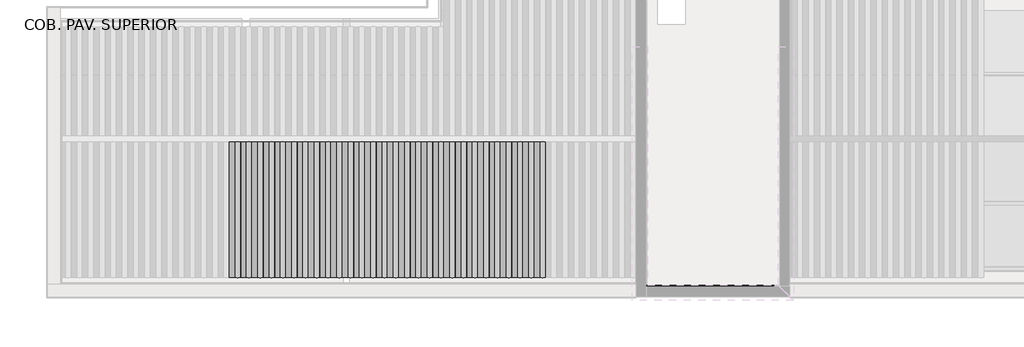
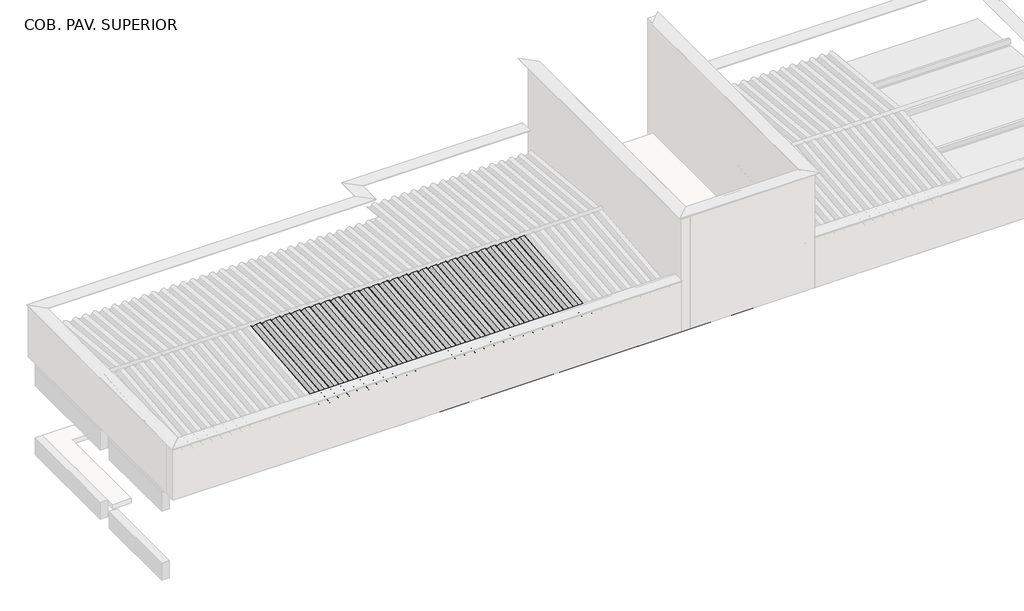
# One storey, part 2 of 7: 38 beams, 9 columns.
"""IFC4 building model written with IfcOpenShell, lengths in millimetres."""

import ifcopenshell
import ifcopenshell.guid

model = None  # the IFC model being written
_history = None  # IfcOwnerHistory: only IFC2X3 demands one
_inside = {}  # id of a spatial element -> (the spatial element, [elements in it])
_under = {}  # id of a project, library or spatial element -> (it, [spatial elements below it])
_declared = {}  # id of a project -> (the project, [libraries it declares])
_typed = {}  # id of a type object -> (the type object, [elements of that type])
_made_of = {}  # id of a material, layer set ... -> (it, [elements and type objects made of it])


def new_model(schema):
    """Start an empty IFC model of exactly this schema.

    Asked for "IFC4X3", IfcOpenShell would pick the latest addendum, in which some entities
    have other attributes; the version numbers below select the first issue.
    IFC2X3 requires an IfcOwnerHistory on every rooted entity: one is made here for all.
    """
    global model, _history
    if schema == "IFC4X3":
        model = ifcopenshell.file(schema_version=(4, 3, 0, 0))
    else:
        model = ifcopenshell.file(schema=schema)
    _inside.clear()
    _under.clear()
    _declared.clear()
    _typed.clear()
    _made_of.clear()
    _history = None
    if model.schema == "IFC2X3":
        org = make("IfcOrganization", Name="unknown")
        user = make(
            "IfcPersonAndOrganization",
            ThePerson=make("IfcPerson", FamilyName="unknown"),
            TheOrganization=org,
        )
        app = make(
            "IfcApplication",
            ApplicationDeveloper=org,
            Version="unknown",
            ApplicationFullName="unknown",
            ApplicationIdentifier="unknown",
        )
        _history = make(
            "IfcOwnerHistory",
            OwningUser=user,
            OwningApplication=app,
            ChangeAction="ADDED",
            CreationDate=0,
        )
    return model


def make(cls, **values):
    """One entity of the class cls with the attributes given. An attribute that is None is left unset."""
    return model.create_entity(
        cls, **{name: value for name, value in values.items() if value is not None}
    )


def rooted(cls, **values):
    """An entity with a GlobalId (a new one), such as an element, a storey or a relation."""
    return make(cls, GlobalId=ifcopenshell.guid.new(), OwnerHistory=_history, **values)


def si_unit(unit_type, name, prefix=None):
    """IfcSIUnit, for example si_unit("LENGTHUNIT", "METRE", prefix="MILLI")."""
    return make("IfcSIUnit", UnitType=unit_type, Prefix=prefix, Name=name)


def assignment(units):
    """IfcUnitAssignment: the units of a project."""
    return None if units is None else make("IfcUnitAssignment", Units=units)


def point(xyz):
    """IfcCartesianPoint."""
    return None if xyz is None else make("IfcCartesianPoint", Coordinates=xyz)


def direction(xyz):
    """IfcDirection."""
    return None if xyz is None else make("IfcDirection", DirectionRatios=xyz)


def frame(location, z_axis=None, x_axis=None):
    """IfcAxis2Placement3D, a coordinate frame: its origin and axes. An axis left out is left unset."""
    return make(
        "IfcAxis2Placement3D",
        Location=point(location),
        Axis=direction(z_axis),
        RefDirection=direction(x_axis),
    )


def frame_2d(location, x_axis=None):
    """IfcAxis2Placement2D, a coordinate frame in the plane: its origin and x axis."""
    return make(
        "IfcAxis2Placement2D", Location=point(location), RefDirection=direction(x_axis)
    )


def origin():
    """The frame at (0, 0, 0) with its axes left unset."""
    return frame((0.0, 0.0, 0.0))


def place(relative_to, where):
    """IfcLocalPlacement: puts the frame where relative to a parent placement (None: the world)."""
    return make(
        "IfcLocalPlacement", PlacementRelTo=relative_to, RelativePlacement=where
    )


def context(
    kind, dimensions, precision=None, world=None, true_north=None, identifier=None
):
    """IfcGeometricRepresentationContext, for example the 3D "Model" context."""
    return make(
        "IfcGeometricRepresentationContext",
        ContextIdentifier=identifier,
        ContextType=kind,
        CoordinateSpaceDimension=dimensions,
        Precision=precision,
        WorldCoordinateSystem=world,
        TrueNorth=true_north,
    )


def project(units=None, contexts=None):
    """IfcProject with its units and contexts."""
    return rooted(
        "IfcProject",
        Name="project",
        RepresentationContexts=contexts,
        UnitsInContext=assignment(units),
    )


def spatial(cls, under=None, at=None, **own):
    """A site, building, storey or space (cls), placed at a placement, below another one or the project."""
    s = rooted(cls, ObjectPlacement=at, **own)
    if under is not None:
        _under.setdefault(under.id(), (under, []))[1].append(s)
    return s


def polyline(points):
    """IfcPolyline through the points."""
    return make("IfcPolyline", Points=[point(p) for p in points])


def circle_curve(where, radius):
    """IfcCircle in the frame where."""
    return make("IfcCircle", Position=where, Radius=radius)


def trimmed(basis, trim1, trim2, sense, master):
    """IfcTrimmedCurve: the piece of a basis curve between two trims."""
    return make(
        "IfcTrimmedCurve",
        BasisCurve=basis,
        Trim1=trim1,
        Trim2=trim2,
        SenseAgreement=sense,
        MasterRepresentation=master,
    )


def segment(curve, same_sense, transition):
    """IfcCompositeCurveSegment."""
    return make(
        "IfcCompositeCurveSegment",
        Transition=transition,
        SameSense=same_sense,
        ParentCurve=curve,
    )


def composite_curve(segments, self_intersect=None):
    """IfcCompositeCurve: segments joined end to end."""
    return make("IfcCompositeCurve", Segments=segments, SelfIntersect=self_intersect)


def outline(outer, holes=None, kind="AREA"):
    """IfcArbitraryClosedProfileDef: a profile drawn as a closed curve; with holes, ...WithVoids."""
    if holes is None:
        return make("IfcArbitraryClosedProfileDef", ProfileType=kind, OuterCurve=outer)
    return make(
        "IfcArbitraryProfileDefWithVoids",
        ProfileType=kind,
        OuterCurve=outer,
        InnerCurves=holes,
    )


def extrude(swept, where, along, depth):
    """IfcExtrudedAreaSolid: the profile swept, set in the frame where, extruded along a direction by depth."""
    return make(
        "IfcExtrudedAreaSolid",
        SweptArea=swept,
        Position=where,
        ExtrudedDirection=direction(along),
        Depth=depth,
    )


def faces_of(points, faces, orient=None, outer=None):
    """IfcFace entities. A face is a list of loops; a loop is a list of indices into points, from 0.

    orient and outer hold one flag for each loop. By default every Orientation is true, the
    first loop of a face is its IfcFaceOuterBound and the others are IfcFaceBound.
    """
    made = []
    for i, loops in enumerate(faces):
        bounds = []
        for j, loop in enumerate(loops):
            is_outer = j == 0 if outer is None else outer[i][j]
            bounds.append(
                make(
                    "IfcFaceOuterBound" if is_outer else "IfcFaceBound",
                    Bound=make("IfcPolyLoop", Polygon=[points[k] for k in loop]),
                    Orientation=True if orient is None else orient[i][j],
                )
            )
        made.append(make("IfcFace", Bounds=bounds))
    return made


def faceted_brep(points, faces, orient=None, outer=None, voids=None):
    """IfcFacetedBrep: a solid bounded by flat faces; with voids (closed shells), ...WithVoids."""
    shared = [point(p) for p in points]
    hull = make("IfcClosedShell", CfsFaces=faces_of(shared, faces, orient, outer))
    if voids is None:
        return make("IfcFacetedBrep", Outer=hull)
    return make(
        "IfcFacetedBrepWithVoids",
        Outer=hull,
        Voids=[
            make(cls, CfsFaces=faces_of(shared, fs, o, b)) for cls, fs, o, b in voids
        ],
    )


def shape(context_of_items, identifier, shape_type, items):
    """IfcShapeRepresentation: the items that make up one representation, for example the "Body"."""
    return make(
        "IfcShapeRepresentation",
        ContextOfItems=context_of_items,
        RepresentationIdentifier=identifier,
        RepresentationType=shape_type,
        Items=items,
    )


def source(mapping_origin, context_of_items, identifier, shape_type, items):
    """IfcRepresentationMap: a shape defined once, which mapped items show again and again."""
    return make(
        "IfcRepresentationMap",
        MappingOrigin=mapping_origin,
        MappedRepresentation=shape(context_of_items, identifier, shape_type, items),
    )


def transform(
    local_origin,
    x_axis=None,
    y_axis=None,
    z_axis=None,
    scale=None,
    scale2=None,
    scale3=None,
    uniform=True,
):
    """IfcCartesianTransformationOperator3D, or its non-uniform kind. x_axis, y_axis, z_axis: its Axis1, 2, 3."""
    if uniform:
        return make(
            "IfcCartesianTransformationOperator3D",
            Axis1=direction(x_axis),
            Axis2=direction(y_axis),
            LocalOrigin=point(local_origin),
            Scale=scale,
            Axis3=direction(z_axis),
        )
    return make(
        "IfcCartesianTransformationOperator3DnonUniform",
        Axis1=direction(x_axis),
        Axis2=direction(y_axis),
        LocalOrigin=point(local_origin),
        Scale=scale,
        Axis3=direction(z_axis),
        Scale2=scale2,
        Scale3=scale3,
    )


def mapped(mapping_source, mapping_target):
    """IfcMappedItem: shows the shape of a source again, moved by a transform."""
    return make(
        "IfcMappedItem", MappingSource=mapping_source, MappingTarget=mapping_target
    )


def made_of(thing, what):
    """Note that an element or type object is made of a material, layer set ...; save() writes the relation."""
    if what is not None:
        _made_of.setdefault(what.id(), (what, []))[1].append(thing)
    return thing


def element(
    cls,
    number,
    at=None,
    inside=None,
    cuts=None,
    type_object=None,
    material=None,
    context=None,
    identifier="Body",
    shape_type=None,
    held_by="IfcProductDefinitionShape",
    body=None,
    shapes=None,
    **own,
):
    """One element of the class cls, such as IfcWall. Its Tag is "e" and its number.

    at: its placement. inside: the storey or other place that contains it. cuts: it is an
    opening in that element (IfcRelVoidsElement). A single representation is given by context,
    identifier, shape_type and body (its items); several are given by shapes. held_by: the class
    of the entity that holds the representations. save() writes the other relations.
    """
    e = rooted(cls, Tag="e%d" % number, ObjectPlacement=at, **own)
    if body is not None:
        shapes = [shape(context, identifier, shape_type, body)]
    if shapes is not None:
        e.Representation = make(held_by, Representations=shapes)
    if inside is not None:
        _inside.setdefault(inside.id(), (inside, []))[1].append(e)
    if cuts is not None:
        rooted(
            "IfcRelVoidsElement", RelatingBuildingElement=cuts, RelatedOpeningElement=e
        )
    if type_object is not None:
        _typed.setdefault(type_object.id(), (type_object, []))[1].append(e)
    return made_of(e, material)


def aggregate(whole, parts):
    """IfcRelAggregates: a whole, such as a stair, and the parts it consists of."""
    return rooted("IfcRelAggregates", RelatingObject=whole, RelatedObjects=parts)


def save(model, path):
    """Write the relations noted so far, then the file.

    IfcRelAggregates (storeys below a building ...), IfcRelContainedInSpatialStructure (elements
    in a storey), IfcRelDefinesByType, IfcRelAssociatesMaterial and IfcRelDeclares: one each for
    every whole, place, type object, material and project.
    """
    for whole, parts in _under.values():
        aggregate(whole, parts)
    for where, things in _inside.values():
        rooted(
            "IfcRelContainedInSpatialStructure",
            RelatedElements=things,
            RelatingStructure=where,
        )
    for kind, things in _typed.values():
        rooted("IfcRelDefinesByType", RelatedObjects=things, RelatingType=kind)
    for what, things in _made_of.values():
        rooted("IfcRelAssociatesMaterial", RelatedObjects=things, RelatingMaterial=what)
    for by, libraries in _declared.values():
        rooted("IfcRelDeclares", RelatingContext=by, RelatedDefinitions=libraries)
    model.write(path)


def column_4db371bd(model_context):
    return source(origin(), model_context, "Body", "SweptSolid", [
        extrude(outline(polyline([(30.0, 80.0), (30.0, -80.0), (-30.0, -80.0), (-30.0, 80.0), (30.0, 80.0)])), frame((0.0, 0.0, 6710.0), z_axis=(0.0, 0.0, 1.0), x_axis=(1.0, 0.0, 0.0)), (0.0, 0.0, 1.0), 660.0),
    ])


def column_e8b88e91(model_context):
    return source(origin(), model_context, "Body", "SweptSolid", [
        extrude(outline(polyline([(30.0, 80.0), (30.0, -80.0), (-30.0, -80.0), (-30.0, 80.0), (30.0, 80.0)])), frame((0.0, 0.0, 6710.0), z_axis=(0.0, 0.0, 1.0), x_axis=(1.0, 0.0, 0.0)), (0.0, 0.0, 1.0), 515.0),
    ])


model = new_model("IFC4")

# Units and contexts
model_context = context("Model", 3, world=origin())
ifc_project = project(units=[si_unit("LENGTHUNIT", "METRE", prefix="MILLI")], contexts=[model_context])

# Site, building, storey
site = spatial("IfcSite", under=ifc_project)
building = spatial("IfcBuilding", under=site)
storey = spatial("IfcBuildingStorey", under=building, Name="COB. PAV. SUPERIOR", Elevation=6650.0)

# Beams
placement = place(None, origin())
element("IfcBeam", 1, ObjectType="Madeira de lei : Berço 6x12cm", at=placement, inside=storey, context=model_context, shape_type="SweptSolid", body=[
    extrude(outline(polyline([(-8679.281307, -9101.268869), (-8679.281307, -9221.268869), (-10679.281307, -9221.268869), (-10679.281307, -9101.268869), (-8679.281307, -9101.268869)])), frame((0.0, 0.0, 6650.0), z_axis=(0.0, 0.0, 1.0), x_axis=(1.0, 0.0, 0.0)), (0.0, 0.0, 1.0), 60.0),
])
element("IfcBeam", 2, ObjectType="Madeira de lei : Berço 6x12cm", at=placement, inside=storey, context=model_context, shape_type="SweptSolid", body=[
    extrude(outline(polyline([(-6679.281307, -9101.268869), (-6679.281307, -9221.268869), (-8679.281307, -9221.268869), (-8679.281307, -9101.268869), (-6679.281307, -9101.268869)])), frame((0.0, 0.0, 6650.0), z_axis=(0.0, 0.0, 1.0), x_axis=(1.0, 0.0, 0.0)), (0.0, 0.0, 1.0), 60.0),
])
element("IfcBeam", 3, ObjectType="Madeira de lei : Berço 6x12cm", at=placement, inside=storey, context=model_context, shape_type="SweptSolid", body=[
    extrude(outline(polyline([(-6679.281307, -10521.818869), (-6679.281307, -10641.818869), (-8679.281307, -10641.818869), (-8679.281307, -10521.818869), (-6679.281307, -10521.818869)])), frame((0.0, 0.0, 6650.0), z_axis=(0.0, 0.0, 1.0), x_axis=(1.0, 0.0, 0.0)), (0.0, 0.0, 1.0), 60.0),
])
element("IfcBeam", 4, ObjectType="Madeira de lei : Berço 6x12cm", at=placement, inside=storey, context=model_context, shape_type="SweptSolid", body=[
    extrude(outline(polyline([(-4679.281307, -9101.268869), (-4679.281307, -9221.268869), (-6679.281307, -9221.268869), (-6679.281307, -9101.268869), (-4679.281307, -9101.268869)])), frame((0.0, 0.0, 6650.0), z_axis=(0.0, 0.0, 1.0), x_axis=(1.0, 0.0, 0.0)), (0.0, 0.0, 1.0), 60.0),
])
element("IfcBeam", 5, ObjectType="Madeira de lei : Berço 6x12cm", at=placement, inside=storey, context=model_context, shape_type="SweptSolid", body=[
    extrude(outline(polyline([(-4679.281307, -10521.818869), (-4679.281307, -10641.818869), (-6679.281307, -10641.818869), (-6679.281307, -10521.818869), (-4679.281307, -10521.818869)])), frame((0.0, 0.0, 6650.0), z_axis=(0.0, 0.0, 1.0), x_axis=(1.0, 0.0, 0.0)), (0.0, 0.0, 1.0), 60.0),
])
element("IfcBeam", 6, ObjectType="Madeira de lei : Berço 6x12cm", at=placement, inside=storey, context=model_context, shape_type="SweptSolid", body=[
    extrude(outline(polyline([(-2679.281307, -9101.268869), (-2679.281307, -9221.268869), (-4679.281307, -9221.268869), (-4679.281307, -9101.268869), (-2679.281307, -9101.268869)])), frame((0.0, 0.0, 6650.0), z_axis=(0.0, 0.0, 1.0), x_axis=(1.0, 0.0, 0.0)), (0.0, 0.0, 1.0), 60.0),
])
element("IfcBeam", 7, ObjectType="Madeira de lei : Berço 6x12cm", at=placement, inside=storey, context=model_context, shape_type="SweptSolid", body=[
    extrude(outline(polyline([(-2679.281307, -10521.818869), (-2679.281307, -10641.818869), (-4679.281307, -10641.818869), (-4679.281307, -10521.818869), (-2679.281307, -10521.818869)])), frame((0.0, 0.0, 6650.0), z_axis=(0.0, 0.0, 1.0), x_axis=(1.0, 0.0, 0.0)), (0.0, 0.0, 1.0), 60.0),
])
element("IfcBeam", 8, ObjectType="Madeira de lei : Berço 6x12cm", at=placement, inside=storey, context=model_context, shape_type="SweptSolid", body=[
    extrude(outline(polyline([(-679.281307, -10521.818869), (-679.281307, -10641.818869), (-2679.281307, -10641.818869), (-2679.281307, -10521.818869), (-679.281307, -10521.818869)])), frame((0.0, 0.0, 6650.0), z_axis=(0.0, 0.0, 1.0), x_axis=(1.0, 0.0, 0.0)), (0.0, 0.0, 1.0), 60.0),
])
element("IfcBeam", 9, ObjectType="Madeira de lei : Berço 6x12cm", at=placement, inside=storey, context=model_context, shape_type="SweptSolid", body=[
    extrude(outline(polyline([(-239.281307, -10521.818869), (-239.281307, -10641.818869), (-679.281307, -10641.818869), (-679.281307, -10521.818869), (-239.281307, -10521.818869)])), frame((0.0, 0.0, 6650.0), z_axis=(0.0, 0.0, 1.0), x_axis=(1.0, 0.0, 0.0)), (0.0, 0.0, 1.0), 60.0),
])
element("IfcBeam", 10, ObjectType="TQS - Viga retangular : 19.0 x 80.0", at=placement, inside=storey, context=model_context, shape_type="Brep", body=[
    faceted_brep([(3049.718693, -10953.5699847, 7250.0), (3049.718693, -11143.5699847, 7250.0), (4178.718693, -11143.5699847, 7250.0), (4178.718693, -10953.5699847, 7250.0), (-6249.181307, -11143.5699847, 6450.0), (-312.281307, -11143.5699847, 6450.0), (-12.281307, -11143.5699847, 6450.0), (4178.718693, -11143.5699847, 6450.0), (3049.718693, -11143.5699847, 6650.0), (2749.718693, -11143.5699847, 6650.0), (2749.718693, -11143.5699847, 7250.0), (-12.281307, -11143.5699847, 7250.0), (-12.281307, -11143.5699847, 6650.0), (-202.281307, -11143.5699847, 6650.0), (-202.281307, -11143.5699847, 7250.0), (-6249.181307, -11143.5699847, 7250.0), (-6249.181307, -10953.5699847, 6450.0), (-312.281307, -10953.5699847, 6450.0), (-202.281307, -10953.5699847, 6450.0), (-12.281307, -10953.5699847, 6450.0), (4178.718693, -10953.5699847, 6450.0), (-6249.181307, -10953.5699847, 7250.0), (-202.281307, -10953.5699847, 7250.0), (-202.281307, -10953.5699847, 6650.0), (-12.281307, -10953.5699847, 6650.0), (-12.281307, -10953.5699847, 7250.0), (2749.718693, -10953.5699847, 7250.0), (2749.718693, -10953.5699847, 6650.0), (3049.718693, -10953.5699847, 6650.0)], [[[0, 1, 2, 3]], [[4, 5, 6, 7, 2, 1, 8, 9, 10, 11, 12, 13, 14, 15]], [[7, 6, 5, 4, 16, 17, 18, 19, 20]], [[20, 19, 18, 17, 16, 21, 22, 23, 24, 25, 26, 27, 28, 0, 3]], [[8, 28, 27, 9]], [[28, 8, 1, 0]], [[9, 27, 26, 10]], [[10, 26, 25, 11]], [[21, 16, 4, 15]], [[3, 2, 7, 20]], [[12, 24, 23, 13]], [[24, 12, 11, 25]], [[13, 23, 22, 14]], [[21, 15, 14, 22]]]),
])
element("IfcBeam", 11, ObjectType="Telha Ondulada : Fibrocimento", at=placement, inside=storey, context=model_context, shape_type="SweptSolid", body=[
    extrude(outline(composite_curve([segment(trimmed(circle_curve(frame_2d((0.0, 66.7939461)), 66.7939461), [point((29.3501489, 6.7939461))], [point((29.3501489, 126.7939461))], True, "CARTESIAN"), True, "CONTINUOUS"), segment(polyline([(29.3501489, 126.7939461), (31.5472154, 131.2853711)]), True, "CONTINUOUS"), segment(trimmed(circle_curve(frame_2d((0.0, 66.7939461)), 71.7939461), [point((31.5472154, 131.2853711))], [point((31.5472154, 2.3025211))], False, "CARTESIAN"), True, "CONTINUOUS"), segment(trimmed(circle_curve(frame_2d((58.7002978, -53.2060539)), 61.7939461), [point((31.5472154, 2.3025211))], [point((31.5472154, -108.7146289))], True, "CARTESIAN"), True, "CONTINUOUS"), segment(polyline([(31.5472154, -108.7146289), (29.3501489, -113.2060539)]), True, "CONTINUOUS"), segment(trimmed(circle_curve(frame_2d((58.7002978, -53.2060539)), 66.7939461), [point((29.3501489, -113.2060539))], [point((29.3501489, 6.7939461))], False, "CARTESIAN"), True, "CONTINUOUS")], self_intersect=False)), frame((-8917.8843743, -10781.9594023, 7394.5315886), z_axis=(0.0, 0.9950371902099894, 0.09950371902099743), x_axis=(0.0, 0.09950371902099743, -0.9950371902099894)), (0.0, 0.0, 1.0), 3017.2295147),
])
element("IfcBeam", 12, ObjectType="Telha Ondulada : Fibrocimento", at=placement, inside=storey, context=model_context, shape_type="SweptSolid", body=[
    extrude(outline(composite_curve([segment(trimmed(circle_curve(frame_2d((0.0, 66.7939461)), 66.7939461), [point((29.3501489, 6.7939461))], [point((29.3501489, 126.7939461))], True, "CARTESIAN"), True, "CONTINUOUS"), segment(polyline([(29.3501489, 126.7939461), (31.5472154, 131.2853711)]), True, "CONTINUOUS"), segment(trimmed(circle_curve(frame_2d((0.0, 66.7939461)), 71.7939461), [point((31.5472154, 131.2853711))], [point((31.5472154, 2.3025211))], False, "CARTESIAN"), True, "CONTINUOUS"), segment(trimmed(circle_curve(frame_2d((58.7002978, -53.2060539)), 61.7939461), [point((31.5472154, 2.3025211))], [point((31.5472154, -108.7146289))], True, "CARTESIAN"), True, "CONTINUOUS"), segment(polyline([(31.5472154, -108.7146289), (29.3501489, -113.2060539)]), True, "CONTINUOUS"), segment(trimmed(circle_curve(frame_2d((58.7002978, -53.2060539)), 66.7939461), [point((29.3501489, -113.2060539))], [point((29.3501489, 6.7939461))], False, "CARTESIAN"), True, "CONTINUOUS")], self_intersect=False)), frame((-8673.3843743, -10781.9594023, 7394.5315886), z_axis=(0.0, 0.9950371902099894, 0.09950371902099743), x_axis=(0.0, 0.09950371902099743, -0.9950371902099894)), (0.0, 0.0, 1.0), 3017.2295147),
])
element("IfcBeam", 13, ObjectType="Telha Ondulada : Fibrocimento", at=placement, inside=storey, context=model_context, shape_type="SweptSolid", body=[
    extrude(outline(composite_curve([segment(trimmed(circle_curve(frame_2d((0.0, 66.7939461)), 66.7939461), [point((29.3501489, 6.7939461))], [point((29.3501489, 126.7939461))], True, "CARTESIAN"), True, "CONTINUOUS"), segment(polyline([(29.3501489, 126.7939461), (31.5472154, 131.2853711)]), True, "CONTINUOUS"), segment(trimmed(circle_curve(frame_2d((0.0, 66.7939461)), 71.7939461), [point((31.5472154, 131.2853711))], [point((31.5472154, 2.3025211))], False, "CARTESIAN"), True, "CONTINUOUS"), segment(trimmed(circle_curve(frame_2d((58.7002978, -53.2060539)), 61.7939461), [point((31.5472154, 2.3025211))], [point((31.5472154, -108.7146289))], True, "CARTESIAN"), True, "CONTINUOUS"), segment(polyline([(31.5472154, -108.7146289), (29.3501489, -113.2060539)]), True, "CONTINUOUS"), segment(trimmed(circle_curve(frame_2d((58.7002978, -53.2060539)), 66.7939461), [point((29.3501489, -113.2060539))], [point((29.3501489, 6.7939461))], False, "CARTESIAN"), True, "CONTINUOUS")], self_intersect=False)), frame((-8428.8843743, -10781.9594023, 7394.5315886), z_axis=(0.0, 0.9950371902099894, 0.0995037190209974), x_axis=(0.0, 0.0995037190209974, -0.9950371902099894)), (0.0, 0.0, 1.0), 3017.2295147),
])
element("IfcBeam", 14, ObjectType="Telha Ondulada : Fibrocimento", at=placement, inside=storey, context=model_context, shape_type="SweptSolid", body=[
    extrude(outline(composite_curve([segment(trimmed(circle_curve(frame_2d((0.0, 66.7939461)), 66.7939461), [point((29.3501489, 6.7939461))], [point((29.3501489, 126.7939461))], True, "CARTESIAN"), True, "CONTINUOUS"), segment(polyline([(29.3501489, 126.7939461), (31.5472154, 131.2853711)]), True, "CONTINUOUS"), segment(trimmed(circle_curve(frame_2d((0.0, 66.7939461)), 71.7939461), [point((31.5472154, 131.2853711))], [point((31.5472154, 2.3025211))], False, "CARTESIAN"), True, "CONTINUOUS"), segment(trimmed(circle_curve(frame_2d((58.7002978, -53.2060539)), 61.7939461), [point((31.5472154, 2.3025211))], [point((31.5472154, -108.7146289))], True, "CARTESIAN"), True, "CONTINUOUS"), segment(polyline([(31.5472154, -108.7146289), (29.3501489, -113.2060539)]), True, "CONTINUOUS"), segment(trimmed(circle_curve(frame_2d((58.7002978, -53.2060539)), 66.7939461), [point((29.3501489, -113.2060539))], [point((29.3501489, 6.7939461))], False, "CARTESIAN"), True, "CONTINUOUS")], self_intersect=False)), frame((-8184.3843743, -10781.9594023, 7394.5315886), z_axis=(0.0, 0.9950371902099894, 0.09950371902099736), x_axis=(0.0, 0.09950371902099736, -0.9950371902099894)), (0.0, 0.0, 1.0), 3017.2295147),
])
element("IfcBeam", 15, ObjectType="Telha Ondulada : Fibrocimento", at=placement, inside=storey, context=model_context, shape_type="SweptSolid", body=[
    extrude(outline(composite_curve([segment(trimmed(circle_curve(frame_2d((0.0, 66.7939461)), 66.7939461), [point((29.3501489, 6.7939461))], [point((29.3501489, 126.7939461))], True, "CARTESIAN"), True, "CONTINUOUS"), segment(polyline([(29.3501489, 126.7939461), (31.5472154, 131.2853711)]), True, "CONTINUOUS"), segment(trimmed(circle_curve(frame_2d((0.0, 66.7939461)), 71.7939461), [point((31.5472154, 131.2853711))], [point((31.5472154, 2.3025211))], False, "CARTESIAN"), True, "CONTINUOUS"), segment(trimmed(circle_curve(frame_2d((58.7002978, -53.2060539)), 61.7939461), [point((31.5472154, 2.3025211))], [point((31.5472154, -108.7146289))], True, "CARTESIAN"), True, "CONTINUOUS"), segment(polyline([(31.5472154, -108.7146289), (29.3501489, -113.2060539)]), True, "CONTINUOUS"), segment(trimmed(circle_curve(frame_2d((58.7002978, -53.2060539)), 66.7939461), [point((29.3501489, -113.2060539))], [point((29.3501489, 6.7939461))], False, "CARTESIAN"), True, "CONTINUOUS")], self_intersect=False)), frame((-7939.8843743, -10781.9594023, 7394.5315886), z_axis=(0.0, 0.9950371902099894, 0.09950371902099743), x_axis=(0.0, 0.09950371902099743, -0.9950371902099894)), (0.0, 0.0, 1.0), 3017.2295147),
])
element("IfcBeam", 16, ObjectType="Telha Ondulada : Fibrocimento", at=placement, inside=storey, context=model_context, shape_type="SweptSolid", body=[
    extrude(outline(composite_curve([segment(trimmed(circle_curve(frame_2d((0.0, 66.7939461)), 66.7939461), [point((29.3501489, 6.7939461))], [point((29.3501489, 126.7939461))], True, "CARTESIAN"), True, "CONTINUOUS"), segment(polyline([(29.3501489, 126.7939461), (31.5472154, 131.2853711)]), True, "CONTINUOUS"), segment(trimmed(circle_curve(frame_2d((0.0, 66.7939461)), 71.7939461), [point((31.5472154, 131.2853711))], [point((31.5472154, 2.3025211))], False, "CARTESIAN"), True, "CONTINUOUS"), segment(trimmed(circle_curve(frame_2d((58.7002978, -53.2060539)), 61.7939461), [point((31.5472154, 2.3025211))], [point((31.5472154, -108.7146289))], True, "CARTESIAN"), True, "CONTINUOUS"), segment(polyline([(31.5472154, -108.7146289), (29.3501489, -113.2060539)]), True, "CONTINUOUS"), segment(trimmed(circle_curve(frame_2d((58.7002978, -53.2060539)), 66.7939461), [point((29.3501489, -113.2060539))], [point((29.3501489, 6.7939461))], False, "CARTESIAN"), True, "CONTINUOUS")], self_intersect=False)), frame((-7695.3843743, -10781.9594023, 7394.5315886), z_axis=(0.0, 0.9950371902099894, 0.09950371902099743), x_axis=(0.0, 0.09950371902099743, -0.9950371902099894)), (0.0, 0.0, 1.0), 3017.2295147),
])
element("IfcBeam", 17, ObjectType="Telha Ondulada : Fibrocimento", at=placement, inside=storey, context=model_context, shape_type="SweptSolid", body=[
    extrude(outline(composite_curve([segment(trimmed(circle_curve(frame_2d((0.0, 66.7939461)), 66.7939461), [point((29.3501489, 6.7939461))], [point((29.3501489, 126.7939461))], True, "CARTESIAN"), True, "CONTINUOUS"), segment(polyline([(29.3501489, 126.7939461), (31.5472154, 131.2853711)]), True, "CONTINUOUS"), segment(trimmed(circle_curve(frame_2d((0.0, 66.7939461)), 71.7939461), [point((31.5472154, 131.2853711))], [point((31.5472154, 2.3025211))], False, "CARTESIAN"), True, "CONTINUOUS"), segment(trimmed(circle_curve(frame_2d((58.7002978, -53.2060539)), 61.7939461), [point((31.5472154, 2.3025211))], [point((31.5472154, -108.7146289))], True, "CARTESIAN"), True, "CONTINUOUS"), segment(polyline([(31.5472154, -108.7146289), (29.3501489, -113.2060539)]), True, "CONTINUOUS"), segment(trimmed(circle_curve(frame_2d((58.7002978, -53.2060539)), 66.7939461), [point((29.3501489, -113.2060539))], [point((29.3501489, 6.7939461))], False, "CARTESIAN"), True, "CONTINUOUS")], self_intersect=False)), frame((-7450.8843743, -10781.9594023, 7394.5315886), z_axis=(0.0, 0.9950371902099894, 0.09950371902099743), x_axis=(0.0, 0.09950371902099743, -0.9950371902099894)), (0.0, 0.0, 1.0), 3017.2295147),
])
element("IfcBeam", 18, ObjectType="Telha Ondulada : Fibrocimento", at=placement, inside=storey, context=model_context, shape_type="SweptSolid", body=[
    extrude(outline(composite_curve([segment(trimmed(circle_curve(frame_2d((0.0, 66.7939461)), 66.7939461), [point((29.3501489, 6.7939461))], [point((29.3501489, 126.7939461))], True, "CARTESIAN"), True, "CONTINUOUS"), segment(polyline([(29.3501489, 126.7939461), (31.5472154, 131.2853711)]), True, "CONTINUOUS"), segment(trimmed(circle_curve(frame_2d((0.0, 66.7939461)), 71.7939461), [point((31.5472154, 131.2853711))], [point((31.5472154, 2.3025211))], False, "CARTESIAN"), True, "CONTINUOUS"), segment(trimmed(circle_curve(frame_2d((58.7002978, -53.2060539)), 61.7939461), [point((31.5472154, 2.3025211))], [point((31.5472154, -108.7146289))], True, "CARTESIAN"), True, "CONTINUOUS"), segment(polyline([(31.5472154, -108.7146289), (29.3501489, -113.2060539)]), True, "CONTINUOUS"), segment(trimmed(circle_curve(frame_2d((58.7002978, -53.2060539)), 66.7939461), [point((29.3501489, -113.2060539))], [point((29.3501489, 6.7939461))], False, "CARTESIAN"), True, "CONTINUOUS")], self_intersect=False)), frame((-7206.3843743, -10781.9594023, 7394.5315886), z_axis=(0.0, 0.9950371902099894, 0.0995037190209974), x_axis=(0.0, 0.0995037190209974, -0.9950371902099894)), (0.0, 0.0, 1.0), 3017.2295147),
])
element("IfcBeam", 19, ObjectType="Telha Ondulada : Fibrocimento", at=placement, inside=storey, context=model_context, shape_type="SweptSolid", body=[
    extrude(outline(composite_curve([segment(trimmed(circle_curve(frame_2d((0.0, 66.7939461)), 66.7939461), [point((29.3501489, 6.7939461))], [point((29.3501489, 126.7939461))], True, "CARTESIAN"), True, "CONTINUOUS"), segment(polyline([(29.3501489, 126.7939461), (31.5472154, 131.2853711)]), True, "CONTINUOUS"), segment(trimmed(circle_curve(frame_2d((0.0, 66.7939461)), 71.7939461), [point((31.5472154, 131.2853711))], [point((31.5472154, 2.3025211))], False, "CARTESIAN"), True, "CONTINUOUS"), segment(trimmed(circle_curve(frame_2d((58.7002978, -53.2060539)), 61.7939461), [point((31.5472154, 2.3025211))], [point((31.5472154, -108.7146289))], True, "CARTESIAN"), True, "CONTINUOUS"), segment(polyline([(31.5472154, -108.7146289), (29.3501489, -113.2060539)]), True, "CONTINUOUS"), segment(trimmed(circle_curve(frame_2d((58.7002978, -53.2060539)), 66.7939461), [point((29.3501489, -113.2060539))], [point((29.3501489, 6.7939461))], False, "CARTESIAN"), True, "CONTINUOUS")], self_intersect=False)), frame((-6961.8843743, -10781.9594023, 7394.5315886), z_axis=(0.0, 0.9950371902099894, 0.0995037190209974), x_axis=(0.0, 0.0995037190209974, -0.9950371902099894)), (0.0, 0.0, 1.0), 3017.2295147),
])
element("IfcBeam", 20, ObjectType="Telha Ondulada : Fibrocimento", at=placement, inside=storey, context=model_context, shape_type="SweptSolid", body=[
    extrude(outline(composite_curve([segment(trimmed(circle_curve(frame_2d((0.0, 66.7939461)), 66.7939461), [point((29.3501489, 6.7939461))], [point((29.3501489, 126.7939461))], True, "CARTESIAN"), True, "CONTINUOUS"), segment(polyline([(29.3501489, 126.7939461), (31.5472154, 131.2853711)]), True, "CONTINUOUS"), segment(trimmed(circle_curve(frame_2d((0.0, 66.7939461)), 71.7939461), [point((31.5472154, 131.2853711))], [point((31.5472154, 2.3025211))], False, "CARTESIAN"), True, "CONTINUOUS"), segment(trimmed(circle_curve(frame_2d((58.7002978, -53.2060539)), 61.7939461), [point((31.5472154, 2.3025211))], [point((31.5472154, -108.7146289))], True, "CARTESIAN"), True, "CONTINUOUS"), segment(polyline([(31.5472154, -108.7146289), (29.3501489, -113.2060539)]), True, "CONTINUOUS"), segment(trimmed(circle_curve(frame_2d((58.7002978, -53.2060539)), 66.7939461), [point((29.3501489, -113.2060539))], [point((29.3501489, 6.7939461))], False, "CARTESIAN"), True, "CONTINUOUS")], self_intersect=False)), frame((-6717.3843743, -10781.9594023, 7394.5315886), z_axis=(0.0, 0.9950371902099894, 0.09950371902099743), x_axis=(0.0, 0.09950371902099743, -0.9950371902099894)), (0.0, 0.0, 1.0), 3017.2295147),
])
element("IfcBeam", 21, ObjectType="Telha Ondulada : Fibrocimento", at=placement, inside=storey, context=model_context, shape_type="SweptSolid", body=[
    extrude(outline(composite_curve([segment(trimmed(circle_curve(frame_2d((0.0, 66.7939461)), 66.7939461), [point((29.3501489, 6.7939461))], [point((29.3501489, 126.7939461))], True, "CARTESIAN"), True, "CONTINUOUS"), segment(polyline([(29.3501489, 126.7939461), (31.5472154, 131.2853711)]), True, "CONTINUOUS"), segment(trimmed(circle_curve(frame_2d((0.0, 66.7939461)), 71.7939461), [point((31.5472154, 131.2853711))], [point((31.5472154, 2.3025211))], False, "CARTESIAN"), True, "CONTINUOUS"), segment(trimmed(circle_curve(frame_2d((58.7002978, -53.2060539)), 61.7939461), [point((31.5472154, 2.3025211))], [point((31.5472154, -108.7146289))], True, "CARTESIAN"), True, "CONTINUOUS"), segment(polyline([(31.5472154, -108.7146289), (29.3501489, -113.2060539)]), True, "CONTINUOUS"), segment(trimmed(circle_curve(frame_2d((58.7002978, -53.2060539)), 66.7939461), [point((29.3501489, -113.2060539))], [point((29.3501489, 6.7939461))], False, "CARTESIAN"), True, "CONTINUOUS")], self_intersect=False)), frame((-6472.8843743, -10781.9594023, 7394.5315886), z_axis=(0.0, 0.9950371902099894, 0.09950371902099743), x_axis=(0.0, 0.09950371902099743, -0.9950371902099894)), (0.0, 0.0, 1.0), 3017.2295147),
])
element("IfcBeam", 22, ObjectType="Telha Ondulada : Fibrocimento", at=placement, inside=storey, context=model_context, shape_type="SweptSolid", body=[
    extrude(outline(composite_curve([segment(trimmed(circle_curve(frame_2d((0.0, 66.7939461)), 66.7939461), [point((29.3501489, 6.7939461))], [point((29.3501489, 126.7939461))], True, "CARTESIAN"), True, "CONTINUOUS"), segment(polyline([(29.3501489, 126.7939461), (31.5472154, 131.2853711)]), True, "CONTINUOUS"), segment(trimmed(circle_curve(frame_2d((0.0, 66.7939461)), 71.7939461), [point((31.5472154, 131.2853711))], [point((31.5472154, 2.3025211))], False, "CARTESIAN"), True, "CONTINUOUS"), segment(trimmed(circle_curve(frame_2d((58.7002978, -53.2060539)), 61.7939461), [point((31.5472154, 2.3025211))], [point((31.5472154, -108.7146289))], True, "CARTESIAN"), True, "CONTINUOUS"), segment(polyline([(31.5472154, -108.7146289), (29.3501489, -113.2060539)]), True, "CONTINUOUS"), segment(trimmed(circle_curve(frame_2d((58.7002978, -53.2060539)), 66.7939461), [point((29.3501489, -113.2060539))], [point((29.3501489, 6.7939461))], False, "CARTESIAN"), True, "CONTINUOUS")], self_intersect=False)), frame((-6228.3843743, -10781.9594023, 7394.5315886), z_axis=(0.0, 0.9950371902099894, 0.09950371902099743), x_axis=(0.0, 0.09950371902099743, -0.9950371902099894)), (0.0, 0.0, 1.0), 3017.2295147),
])
element("IfcBeam", 23, ObjectType="Telha Ondulada : Fibrocimento", at=placement, inside=storey, context=model_context, shape_type="SweptSolid", body=[
    extrude(outline(composite_curve([segment(trimmed(circle_curve(frame_2d((0.0, 66.7939461)), 66.7939461), [point((29.3501489, 6.7939461))], [point((29.3501489, 126.7939461))], True, "CARTESIAN"), True, "CONTINUOUS"), segment(polyline([(29.3501489, 126.7939461), (31.5472154, 131.2853711)]), True, "CONTINUOUS"), segment(trimmed(circle_curve(frame_2d((0.0, 66.7939461)), 71.7939461), [point((31.5472154, 131.2853711))], [point((31.5472154, 2.3025211))], False, "CARTESIAN"), True, "CONTINUOUS"), segment(trimmed(circle_curve(frame_2d((58.7002978, -53.2060539)), 61.7939461), [point((31.5472154, 2.3025211))], [point((31.5472154, -108.7146289))], True, "CARTESIAN"), True, "CONTINUOUS"), segment(polyline([(31.5472154, -108.7146289), (29.3501489, -113.2060539)]), True, "CONTINUOUS"), segment(trimmed(circle_curve(frame_2d((58.7002978, -53.2060539)), 66.7939461), [point((29.3501489, -113.2060539))], [point((29.3501489, 6.7939461))], False, "CARTESIAN"), True, "CONTINUOUS")], self_intersect=False)), frame((-5983.8843743, -10781.9594023, 7394.5315886), z_axis=(0.0, 0.9950371902099894, 0.09950371902099743), x_axis=(0.0, 0.09950371902099743, -0.9950371902099894)), (0.0, 0.0, 1.0), 3017.2295147),
])
element("IfcBeam", 24, ObjectType="Telha Ondulada : Fibrocimento", at=placement, inside=storey, context=model_context, shape_type="SweptSolid", body=[
    extrude(outline(composite_curve([segment(trimmed(circle_curve(frame_2d((0.0, 66.7939461)), 66.7939461), [point((29.3501489, 6.7939461))], [point((29.3501489, 126.7939461))], True, "CARTESIAN"), True, "CONTINUOUS"), segment(polyline([(29.3501489, 126.7939461), (31.5472154, 131.2853711)]), True, "CONTINUOUS"), segment(trimmed(circle_curve(frame_2d((0.0, 66.7939461)), 71.7939461), [point((31.5472154, 131.2853711))], [point((31.5472154, 2.3025211))], False, "CARTESIAN"), True, "CONTINUOUS"), segment(trimmed(circle_curve(frame_2d((58.7002978, -53.2060539)), 61.7939461), [point((31.5472154, 2.3025211))], [point((31.5472154, -108.7146289))], True, "CARTESIAN"), True, "CONTINUOUS"), segment(polyline([(31.5472154, -108.7146289), (29.3501489, -113.2060539)]), True, "CONTINUOUS"), segment(trimmed(circle_curve(frame_2d((58.7002978, -53.2060539)), 66.7939461), [point((29.3501489, -113.2060539))], [point((29.3501489, 6.7939461))], False, "CARTESIAN"), True, "CONTINUOUS")], self_intersect=False)), frame((-5739.3843743, -10781.9594023, 7394.5315886), z_axis=(0.0, 0.9950371902099894, 0.0995037190209974), x_axis=(0.0, 0.0995037190209974, -0.9950371902099894)), (0.0, 0.0, 1.0), 3017.2295147),
])
element("IfcBeam", 25, ObjectType="Telha Ondulada : Fibrocimento", at=placement, inside=storey, context=model_context, shape_type="SweptSolid", body=[
    extrude(outline(composite_curve([segment(trimmed(circle_curve(frame_2d((0.0, 66.7939461)), 66.7939461), [point((29.3501489, 6.7939461))], [point((29.3501489, 126.7939461))], True, "CARTESIAN"), True, "CONTINUOUS"), segment(polyline([(29.3501489, 126.7939461), (31.5472154, 131.2853711)]), True, "CONTINUOUS"), segment(trimmed(circle_curve(frame_2d((0.0, 66.7939461)), 71.7939461), [point((31.5472154, 131.2853711))], [point((31.5472154, 2.3025211))], False, "CARTESIAN"), True, "CONTINUOUS"), segment(trimmed(circle_curve(frame_2d((58.7002978, -53.2060539)), 61.7939461), [point((31.5472154, 2.3025211))], [point((31.5472154, -108.7146289))], True, "CARTESIAN"), True, "CONTINUOUS"), segment(polyline([(31.5472154, -108.7146289), (29.3501489, -113.2060539)]), True, "CONTINUOUS"), segment(trimmed(circle_curve(frame_2d((58.7002978, -53.2060539)), 66.7939461), [point((29.3501489, -113.2060539))], [point((29.3501489, 6.7939461))], False, "CARTESIAN"), True, "CONTINUOUS")], self_intersect=False)), frame((-5494.8843743, -10781.9594023, 7394.5315886), z_axis=(0.0, 0.9950371902099894, 0.0995037190209974), x_axis=(0.0, 0.0995037190209974, -0.9950371902099894)), (0.0, 0.0, 1.0), 3017.2295147),
])
element("IfcBeam", 26, ObjectType="Telha Ondulada : Fibrocimento", at=placement, inside=storey, context=model_context, shape_type="SweptSolid", body=[
    extrude(outline(composite_curve([segment(trimmed(circle_curve(frame_2d((0.0, 66.7939461)), 66.7939461), [point((29.3501489, 6.7939461))], [point((29.3501489, 126.7939461))], True, "CARTESIAN"), True, "CONTINUOUS"), segment(polyline([(29.3501489, 126.7939461), (31.5472154, 131.2853711)]), True, "CONTINUOUS"), segment(trimmed(circle_curve(frame_2d((0.0, 66.7939461)), 71.7939461), [point((31.5472154, 131.2853711))], [point((31.5472154, 2.3025211))], False, "CARTESIAN"), True, "CONTINUOUS"), segment(trimmed(circle_curve(frame_2d((58.7002978, -53.2060539)), 61.7939461), [point((31.5472154, 2.3025211))], [point((31.5472154, -108.7146289))], True, "CARTESIAN"), True, "CONTINUOUS"), segment(polyline([(31.5472154, -108.7146289), (29.3501489, -113.2060539)]), True, "CONTINUOUS"), segment(trimmed(circle_curve(frame_2d((58.7002978, -53.2060539)), 66.7939461), [point((29.3501489, -113.2060539))], [point((29.3501489, 6.7939461))], False, "CARTESIAN"), True, "CONTINUOUS")], self_intersect=False)), frame((-5250.3843743, -10781.9594023, 7394.5315886), z_axis=(0.0, 0.9950371902099894, 0.09950371902099736), x_axis=(0.0, 0.09950371902099736, -0.9950371902099894)), (0.0, 0.0, 1.0), 3017.2295147),
])
element("IfcBeam", 27, ObjectType="Telha Ondulada : Fibrocimento", at=placement, inside=storey, context=model_context, shape_type="SweptSolid", body=[
    extrude(outline(composite_curve([segment(trimmed(circle_curve(frame_2d((0.0, 66.7939461)), 66.7939461), [point((29.3501489, 6.7939461))], [point((29.3501489, 126.7939461))], True, "CARTESIAN"), True, "CONTINUOUS"), segment(polyline([(29.3501489, 126.7939461), (31.5472154, 131.2853711)]), True, "CONTINUOUS"), segment(trimmed(circle_curve(frame_2d((0.0, 66.7939461)), 71.7939461), [point((31.5472154, 131.2853711))], [point((31.5472154, 2.3025211))], False, "CARTESIAN"), True, "CONTINUOUS"), segment(trimmed(circle_curve(frame_2d((58.7002978, -53.2060539)), 61.7939461), [point((31.5472154, 2.3025211))], [point((31.5472154, -108.7146289))], True, "CARTESIAN"), True, "CONTINUOUS"), segment(polyline([(31.5472154, -108.7146289), (29.3501489, -113.2060539)]), True, "CONTINUOUS"), segment(trimmed(circle_curve(frame_2d((58.7002978, -53.2060539)), 66.7939461), [point((29.3501489, -113.2060539))], [point((29.3501489, 6.7939461))], False, "CARTESIAN"), True, "CONTINUOUS")], self_intersect=False)), frame((-5005.8843743, -10781.9594023, 7394.5315886), z_axis=(0.0, 0.9950371902099894, 0.09950371902099743), x_axis=(0.0, 0.09950371902099743, -0.9950371902099894)), (0.0, 0.0, 1.0), 3017.2295147),
])
element("IfcBeam", 28, ObjectType="Telha Ondulada : Fibrocimento", at=placement, inside=storey, context=model_context, shape_type="SweptSolid", body=[
    extrude(outline(composite_curve([segment(trimmed(circle_curve(frame_2d((0.0, 66.7939461)), 66.7939461), [point((29.3501489, 6.7939461))], [point((29.3501489, 126.7939461))], True, "CARTESIAN"), True, "CONTINUOUS"), segment(polyline([(29.3501489, 126.7939461), (31.5472154, 131.2853711)]), True, "CONTINUOUS"), segment(trimmed(circle_curve(frame_2d((0.0, 66.7939461)), 71.7939461), [point((31.5472154, 131.2853711))], [point((31.5472154, 2.3025211))], False, "CARTESIAN"), True, "CONTINUOUS"), segment(trimmed(circle_curve(frame_2d((58.7002978, -53.2060539)), 61.7939461), [point((31.5472154, 2.3025211))], [point((31.5472154, -108.7146289))], True, "CARTESIAN"), True, "CONTINUOUS"), segment(polyline([(31.5472154, -108.7146289), (29.3501489, -113.2060539)]), True, "CONTINUOUS"), segment(trimmed(circle_curve(frame_2d((58.7002978, -53.2060539)), 66.7939461), [point((29.3501489, -113.2060539))], [point((29.3501489, 6.7939461))], False, "CARTESIAN"), True, "CONTINUOUS")], self_intersect=False)), frame((-4761.3843743, -10781.9594023, 7394.5315886), z_axis=(0.0, 0.9950371902099894, 0.09950371902099743), x_axis=(0.0, 0.09950371902099743, -0.9950371902099894)), (0.0, 0.0, 1.0), 3017.2295147),
])
element("IfcBeam", 29, ObjectType="Telha Ondulada : Fibrocimento", at=placement, inside=storey, context=model_context, shape_type="SweptSolid", body=[
    extrude(outline(composite_curve([segment(trimmed(circle_curve(frame_2d((0.0, 66.7939461)), 66.7939461), [point((29.3501489, 6.7939461))], [point((29.3501489, 126.7939461))], True, "CARTESIAN"), True, "CONTINUOUS"), segment(polyline([(29.3501489, 126.7939461), (31.5472154, 131.2853711)]), True, "CONTINUOUS"), segment(trimmed(circle_curve(frame_2d((0.0, 66.7939461)), 71.7939461), [point((31.5472154, 131.2853711))], [point((31.5472154, 2.3025211))], False, "CARTESIAN"), True, "CONTINUOUS"), segment(trimmed(circle_curve(frame_2d((58.7002978, -53.2060539)), 61.7939461), [point((31.5472154, 2.3025211))], [point((31.5472154, -108.7146289))], True, "CARTESIAN"), True, "CONTINUOUS"), segment(polyline([(31.5472154, -108.7146289), (29.3501489, -113.2060539)]), True, "CONTINUOUS"), segment(trimmed(circle_curve(frame_2d((58.7002978, -53.2060539)), 66.7939461), [point((29.3501489, -113.2060539))], [point((29.3501489, 6.7939461))], False, "CARTESIAN"), True, "CONTINUOUS")], self_intersect=False)), frame((-4516.8843743, -10781.9594023, 7394.5315886), z_axis=(0.0, 0.9950371902099894, 0.09950371902099743), x_axis=(0.0, 0.09950371902099743, -0.9950371902099894)), (0.0, 0.0, 1.0), 3017.2295147),
])
element("IfcBeam", 30, ObjectType="Telha Ondulada : Fibrocimento", at=placement, inside=storey, context=model_context, shape_type="SweptSolid", body=[
    extrude(outline(composite_curve([segment(trimmed(circle_curve(frame_2d((0.0, 66.7939461)), 66.7939461), [point((29.3501489, 6.7939461))], [point((29.3501489, 126.7939461))], True, "CARTESIAN"), True, "CONTINUOUS"), segment(polyline([(29.3501489, 126.7939461), (31.5472154, 131.2853711)]), True, "CONTINUOUS"), segment(trimmed(circle_curve(frame_2d((0.0, 66.7939461)), 71.7939461), [point((31.5472154, 131.2853711))], [point((31.5472154, 2.3025211))], False, "CARTESIAN"), True, "CONTINUOUS"), segment(trimmed(circle_curve(frame_2d((58.7002978, -53.2060539)), 61.7939461), [point((31.5472154, 2.3025211))], [point((31.5472154, -108.7146289))], True, "CARTESIAN"), True, "CONTINUOUS"), segment(polyline([(31.5472154, -108.7146289), (29.3501489, -113.2060539)]), True, "CONTINUOUS"), segment(trimmed(circle_curve(frame_2d((58.7002978, -53.2060539)), 66.7939461), [point((29.3501489, -113.2060539))], [point((29.3501489, 6.7939461))], False, "CARTESIAN"), True, "CONTINUOUS")], self_intersect=False)), frame((-4272.3843743, -10781.9594023, 7394.5315886), z_axis=(0.0, 0.9950371902099894, 0.0995037190209974), x_axis=(0.0, 0.0995037190209974, -0.9950371902099894)), (0.0, 0.0, 1.0), 3017.2295147),
])
element("IfcBeam", 31, ObjectType="Telha Ondulada : Fibrocimento", at=placement, inside=storey, context=model_context, shape_type="SweptSolid", body=[
    extrude(outline(composite_curve([segment(trimmed(circle_curve(frame_2d((0.0, 66.7939461)), 66.7939461), [point((29.3501489, 6.7939461))], [point((29.3501489, 126.7939461))], True, "CARTESIAN"), True, "CONTINUOUS"), segment(polyline([(29.3501489, 126.7939461), (31.5472154, 131.2853711)]), True, "CONTINUOUS"), segment(trimmed(circle_curve(frame_2d((0.0, 66.7939461)), 71.7939461), [point((31.5472154, 131.2853711))], [point((31.5472154, 2.3025211))], False, "CARTESIAN"), True, "CONTINUOUS"), segment(trimmed(circle_curve(frame_2d((58.7002978, -53.2060539)), 61.7939461), [point((31.5472154, 2.3025211))], [point((31.5472154, -108.7146289))], True, "CARTESIAN"), True, "CONTINUOUS"), segment(polyline([(31.5472154, -108.7146289), (29.3501489, -113.2060539)]), True, "CONTINUOUS"), segment(trimmed(circle_curve(frame_2d((58.7002978, -53.2060539)), 66.7939461), [point((29.3501489, -113.2060539))], [point((29.3501489, 6.7939461))], False, "CARTESIAN"), True, "CONTINUOUS")], self_intersect=False)), frame((-4027.8843743, -10781.9594023, 7394.5315886), z_axis=(0.0, 0.9950371902099894, 0.0995037190209974), x_axis=(0.0, 0.0995037190209974, -0.9950371902099894)), (0.0, 0.0, 1.0), 3017.2295147),
])
element("IfcBeam", 32, ObjectType="Telha Ondulada : Fibrocimento", at=placement, inside=storey, context=model_context, shape_type="SweptSolid", body=[
    extrude(outline(composite_curve([segment(trimmed(circle_curve(frame_2d((0.0, 66.7939461)), 66.7939461), [point((29.3501489, 6.7939461))], [point((29.3501489, 126.7939461))], True, "CARTESIAN"), True, "CONTINUOUS"), segment(polyline([(29.3501489, 126.7939461), (31.5472154, 131.2853711)]), True, "CONTINUOUS"), segment(trimmed(circle_curve(frame_2d((0.0, 66.7939461)), 71.7939461), [point((31.5472154, 131.2853711))], [point((31.5472154, 2.3025211))], False, "CARTESIAN"), True, "CONTINUOUS"), segment(trimmed(circle_curve(frame_2d((58.7002978, -53.2060539)), 61.7939461), [point((31.5472154, 2.3025211))], [point((31.5472154, -108.7146289))], True, "CARTESIAN"), True, "CONTINUOUS"), segment(polyline([(31.5472154, -108.7146289), (29.3501489, -113.2060539)]), True, "CONTINUOUS"), segment(trimmed(circle_curve(frame_2d((58.7002978, -53.2060539)), 66.7939461), [point((29.3501489, -113.2060539))], [point((29.3501489, 6.7939461))], False, "CARTESIAN"), True, "CONTINUOUS")], self_intersect=False)), frame((-3783.3843743, -10781.9594023, 7394.5315886), z_axis=(0.0, 0.9950371902099894, 0.09950371902099743), x_axis=(0.0, 0.09950371902099743, -0.9950371902099894)), (0.0, 0.0, 1.0), 3017.2295147),
])
element("IfcBeam", 33, ObjectType="Telha Ondulada : Fibrocimento", at=placement, inside=storey, context=model_context, shape_type="SweptSolid", body=[
    extrude(outline(composite_curve([segment(trimmed(circle_curve(frame_2d((0.0, 66.7939461)), 66.7939461), [point((29.3501489, 6.7939461))], [point((29.3501489, 126.7939461))], True, "CARTESIAN"), True, "CONTINUOUS"), segment(polyline([(29.3501489, 126.7939461), (31.5472154, 131.2853711)]), True, "CONTINUOUS"), segment(trimmed(circle_curve(frame_2d((0.0, 66.7939461)), 71.7939461), [point((31.5472154, 131.2853711))], [point((31.5472154, 2.3025211))], False, "CARTESIAN"), True, "CONTINUOUS"), segment(trimmed(circle_curve(frame_2d((58.7002978, -53.2060539)), 61.7939461), [point((31.5472154, 2.3025211))], [point((31.5472154, -108.7146289))], True, "CARTESIAN"), True, "CONTINUOUS"), segment(polyline([(31.5472154, -108.7146289), (29.3501489, -113.2060539)]), True, "CONTINUOUS"), segment(trimmed(circle_curve(frame_2d((58.7002978, -53.2060539)), 66.7939461), [point((29.3501489, -113.2060539))], [point((29.3501489, 6.7939461))], False, "CARTESIAN"), True, "CONTINUOUS")], self_intersect=False)), frame((-3538.8843743, -10781.9594023, 7394.5315886), z_axis=(0.0, 0.9950371902099894, 0.09950371902099743), x_axis=(0.0, 0.09950371902099743, -0.9950371902099894)), (0.0, 0.0, 1.0), 3017.2295147),
])
element("IfcBeam", 34, ObjectType="Telha Ondulada : Fibrocimento", at=placement, inside=storey, context=model_context, shape_type="SweptSolid", body=[
    extrude(outline(composite_curve([segment(trimmed(circle_curve(frame_2d((0.0, 66.7939461)), 66.7939461), [point((29.3501489, 6.7939461))], [point((29.3501489, 126.7939461))], True, "CARTESIAN"), True, "CONTINUOUS"), segment(polyline([(29.3501489, 126.7939461), (31.5472154, 131.2853711)]), True, "CONTINUOUS"), segment(trimmed(circle_curve(frame_2d((0.0, 66.7939461)), 71.7939461), [point((31.5472154, 131.2853711))], [point((31.5472154, 2.3025211))], False, "CARTESIAN"), True, "CONTINUOUS"), segment(trimmed(circle_curve(frame_2d((58.7002978, -53.2060539)), 61.7939461), [point((31.5472154, 2.3025211))], [point((31.5472154, -108.7146289))], True, "CARTESIAN"), True, "CONTINUOUS"), segment(polyline([(31.5472154, -108.7146289), (29.3501489, -113.2060539)]), True, "CONTINUOUS"), segment(trimmed(circle_curve(frame_2d((58.7002978, -53.2060539)), 66.7939461), [point((29.3501489, -113.2060539))], [point((29.3501489, 6.7939461))], False, "CARTESIAN"), True, "CONTINUOUS")], self_intersect=False)), frame((-3294.3843743, -10781.9594023, 7394.5315886), z_axis=(0.0, 0.9950371902099894, 0.09950371902099743), x_axis=(0.0, 0.09950371902099743, -0.9950371902099894)), (0.0, 0.0, 1.0), 3017.2295147),
])
element("IfcBeam", 35, ObjectType="Telha Ondulada : Fibrocimento", at=placement, inside=storey, context=model_context, shape_type="SweptSolid", body=[
    extrude(outline(composite_curve([segment(trimmed(circle_curve(frame_2d((0.0, 66.7939461)), 66.7939461), [point((29.3501489, 6.7939461))], [point((29.3501489, 126.7939461))], True, "CARTESIAN"), True, "CONTINUOUS"), segment(polyline([(29.3501489, 126.7939461), (31.5472154, 131.2853711)]), True, "CONTINUOUS"), segment(trimmed(circle_curve(frame_2d((0.0, 66.7939461)), 71.7939461), [point((31.5472154, 131.2853711))], [point((31.5472154, 2.3025211))], False, "CARTESIAN"), True, "CONTINUOUS"), segment(trimmed(circle_curve(frame_2d((58.7002978, -53.2060539)), 61.7939461), [point((31.5472154, 2.3025211))], [point((31.5472154, -108.7146289))], True, "CARTESIAN"), True, "CONTINUOUS"), segment(polyline([(31.5472154, -108.7146289), (29.3501489, -113.2060539)]), True, "CONTINUOUS"), segment(trimmed(circle_curve(frame_2d((58.7002978, -53.2060539)), 66.7939461), [point((29.3501489, -113.2060539))], [point((29.3501489, 6.7939461))], False, "CARTESIAN"), True, "CONTINUOUS")], self_intersect=False)), frame((-3049.8843743, -10781.9594023, 7394.5315886), z_axis=(0.0, 0.9950371902099894, 0.0995037190209974), x_axis=(0.0, 0.0995037190209974, -0.9950371902099894)), (0.0, 0.0, 1.0), 3017.2295147),
])
element("IfcBeam", 36, ObjectType="Telha Ondulada : Fibrocimento", at=placement, inside=storey, context=model_context, shape_type="SweptSolid", body=[
    extrude(outline(composite_curve([segment(trimmed(circle_curve(frame_2d((0.0, 66.7939461)), 66.7939461), [point((29.3501489, 6.7939461))], [point((29.3501489, 126.7939461))], True, "CARTESIAN"), True, "CONTINUOUS"), segment(polyline([(29.3501489, 126.7939461), (31.5472154, 131.2853711)]), True, "CONTINUOUS"), segment(trimmed(circle_curve(frame_2d((0.0, 66.7939461)), 71.7939461), [point((31.5472154, 131.2853711))], [point((31.5472154, 2.3025211))], False, "CARTESIAN"), True, "CONTINUOUS"), segment(trimmed(circle_curve(frame_2d((58.7002978, -53.2060539)), 61.7939461), [point((31.5472154, 2.3025211))], [point((31.5472154, -108.7146289))], True, "CARTESIAN"), True, "CONTINUOUS"), segment(polyline([(31.5472154, -108.7146289), (29.3501489, -113.2060539)]), True, "CONTINUOUS"), segment(trimmed(circle_curve(frame_2d((58.7002978, -53.2060539)), 66.7939461), [point((29.3501489, -113.2060539))], [point((29.3501489, 6.7939461))], False, "CARTESIAN"), True, "CONTINUOUS")], self_intersect=False)), frame((-2805.3843743, -10781.9594023, 7394.5315886), z_axis=(0.0, 0.9950371902099894, 0.09950371902099736), x_axis=(0.0, 0.09950371902099736, -0.9950371902099894)), (0.0, 0.0, 1.0), 3017.2295147),
])
element("IfcBeam", 37, ObjectType="Telha Ondulada : Fibrocimento", at=placement, inside=storey, context=model_context, shape_type="SweptSolid", body=[
    extrude(outline(composite_curve([segment(trimmed(circle_curve(frame_2d((0.0, 66.7939461)), 66.7939461), [point((29.3501489, 6.7939461))], [point((29.3501489, 126.7939461))], True, "CARTESIAN"), True, "CONTINUOUS"), segment(polyline([(29.3501489, 126.7939461), (31.5472154, 131.2853711)]), True, "CONTINUOUS"), segment(trimmed(circle_curve(frame_2d((0.0, 66.7939461)), 71.7939461), [point((31.5472154, 131.2853711))], [point((31.5472154, 2.3025211))], False, "CARTESIAN"), True, "CONTINUOUS"), segment(trimmed(circle_curve(frame_2d((58.7002978, -53.2060539)), 61.7939461), [point((31.5472154, 2.3025211))], [point((31.5472154, -108.7146289))], True, "CARTESIAN"), True, "CONTINUOUS"), segment(polyline([(31.5472154, -108.7146289), (29.3501489, -113.2060539)]), True, "CONTINUOUS"), segment(trimmed(circle_curve(frame_2d((58.7002978, -53.2060539)), 66.7939461), [point((29.3501489, -113.2060539))], [point((29.3501489, 6.7939461))], False, "CARTESIAN"), True, "CONTINUOUS")], self_intersect=False)), frame((-2560.8843743, -10781.9594023, 7394.5315886), z_axis=(0.0, 0.9950371902099894, 0.09950371902099736), x_axis=(0.0, 0.09950371902099736, -0.9950371902099894)), (0.0, 0.0, 1.0), 3017.2295147),
])
element("IfcBeam", 38, ObjectType="Telha Ondulada : Fibrocimento", at=placement, inside=storey, context=model_context, shape_type="SweptSolid", body=[
    extrude(outline(composite_curve([segment(trimmed(circle_curve(frame_2d((0.0, 66.7939461)), 66.7939461), [point((29.3501489, 6.7939461))], [point((29.3501489, 126.7939461))], True, "CARTESIAN"), True, "CONTINUOUS"), segment(polyline([(29.3501489, 126.7939461), (31.5472154, 131.2853711)]), True, "CONTINUOUS"), segment(trimmed(circle_curve(frame_2d((0.0, 66.7939461)), 71.7939461), [point((31.5472154, 131.2853711))], [point((31.5472154, 2.3025211))], False, "CARTESIAN"), True, "CONTINUOUS"), segment(trimmed(circle_curve(frame_2d((58.7002978, -53.2060539)), 61.7939461), [point((31.5472154, 2.3025211))], [point((31.5472154, -108.7146289))], True, "CARTESIAN"), True, "CONTINUOUS"), segment(polyline([(31.5472154, -108.7146289), (29.3501489, -113.2060539)]), True, "CONTINUOUS"), segment(trimmed(circle_curve(frame_2d((58.7002978, -53.2060539)), 66.7939461), [point((29.3501489, -113.2060539))], [point((29.3501489, 6.7939461))], False, "CARTESIAN"), True, "CONTINUOUS")], self_intersect=False)), frame((-2316.3843743, -10781.9594023, 7394.5315886), z_axis=(0.0, 0.9950371902099894, 0.09950371902099743), x_axis=(0.0, 0.09950371902099743, -0.9950371902099894)), (0.0, 0.0, 1.0), 3017.2295147),
])

# Columns
column_shape = column_4db371bd(model_context)
element("IfcColumn", 39, ObjectType="Madeira de lei-Coluna : Pontalete 6X16cm", at=placement, inside=storey, context=model_context, shape_type="MappedRepresentation", body=[
    mapped(column_shape, transform((-9679.281307, -9161.268869, 0.0), x_axis=(0.0, 1.0, 0.0), y_axis=(-1.0, 0.0, 0.0), z_axis=(0.0, 0.0, 1.0))),
])
element("IfcColumn", 40, ObjectType="Madeira de lei-Coluna : Pontalete 6X16cm", at=placement, inside=storey, context=model_context, shape_type="MappedRepresentation", body=[
    mapped(column_shape, transform((-7679.281307, -9161.268869, 0.0), x_axis=(0.0, 1.0, 0.0), y_axis=(-1.0, 0.0, 0.0), z_axis=(0.0, 0.0, 1.0))),
])
element("IfcColumn", 41, ObjectType="Madeira de lei-Coluna : Pontalete 6X16cm", at=placement, inside=storey, context=model_context, shape_type="MappedRepresentation", body=[
    mapped(column_shape, transform((-5679.281307, -9161.268869, 0.0), x_axis=(0.0, 1.0, 0.0), y_axis=(-1.0, 0.0, 0.0), z_axis=(0.0, 0.0, 1.0))),
])
element("IfcColumn", 42, ObjectType="Madeira de lei-Coluna : Pontalete 6X16cm", at=placement, inside=storey, context=model_context, shape_type="MappedRepresentation", body=[
    mapped(column_shape, transform((-3679.281307, -9161.268869, 0.0), x_axis=(0.0, 1.0, 0.0), y_axis=(-1.0, 0.0, 0.0), z_axis=(0.0, 0.0, 1.0))),
])
column_2_shape = column_e8b88e91(model_context)
element("IfcColumn", 43, ObjectType="Madeira de lei-Coluna : Pontalete 6X16cm", at=placement, inside=storey, context=model_context, shape_type="MappedRepresentation", body=[
    mapped(column_2_shape, transform((-7679.281307, -10581.818869, 0.0), x_axis=(0.0, 1.0, 0.0), y_axis=(-1.0, 0.0, 0.0), z_axis=(0.0, 0.0, 1.0))),
])
element("IfcColumn", 44, ObjectType="Madeira de lei-Coluna : Pontalete 6X16cm", at=placement, inside=storey, context=model_context, shape_type="MappedRepresentation", body=[
    mapped(column_2_shape, transform((-5679.281307, -10581.818869, 0.0), x_axis=(0.0, 1.0, 0.0), y_axis=(-1.0, 0.0, 0.0), z_axis=(0.0, 0.0, 1.0))),
])
element("IfcColumn", 45, ObjectType="Madeira de lei-Coluna : Pontalete 6X16cm", at=placement, inside=storey, context=model_context, shape_type="MappedRepresentation", body=[
    mapped(column_2_shape, transform((-3679.281307, -10581.818869, 0.0), x_axis=(0.0, 1.0, 0.0), y_axis=(-1.0, 0.0, 0.0), z_axis=(0.0, 0.0, 1.0))),
])
element("IfcColumn", 46, ObjectType="Madeira de lei-Coluna : Pontalete 6X16cm", at=placement, inside=storey, context=model_context, shape_type="MappedRepresentation", body=[
    mapped(column_2_shape, transform((-1679.281307, -10581.818869, 0.0), x_axis=(0.0, 1.0, 0.0), y_axis=(-1.0, 0.0, 0.0), z_axis=(0.0, 0.0, 1.0))),
])
element("IfcColumn", 47, ObjectType="TQS - Pilar retangular : 19.0 x 19.0", at=placement, inside=storey, context=model_context, shape_type="Brep", body=[
    faceted_brep([(-202.281307, -10953.5699847, 6650.0), (-12.281307, -10953.5699847, 6650.0), (-12.281307, -11143.5699847, 6650.0), (-202.281307, -11143.5699847, 6650.0), (-202.281307, -10953.5699847, 8750.0), (-62.281307, -10953.5699847, 8750.0), (-12.281307, -10953.5699847, 8750.0), (-12.281307, -10953.5699847, 7250.0), (-12.281307, -10953.5699847, 7050.0), (-202.281307, -10953.5699847, 7050.0), (-202.281307, -10953.5699847, 7250.0), (-202.281307, -10953.5699847, 8300.0), (-12.281307, -11143.5699847, 8750.0), (-12.281307, -11143.5699847, 7250.0), (-202.281307, -11143.5699847, 8750.0), (-202.281307, -11143.5699847, 7250.0)], [[[0, 1, 2, 3]], [[4, 5, 6, 7, 8, 1, 0, 9, 10, 11]], [[6, 12, 13, 2, 1, 8, 7]], [[12, 14, 15, 3, 2, 13]], [[14, 4, 11, 10, 9, 0, 3, 15]], [[4, 14, 12, 6, 5]]]),
])

save(model, "model.ifc")

# Revit data of these elements
# Type "Madeira de lei : Berço 6x12cm"
#   A = 0.02 m²
#   Length [instance default] = 1.524 m
#   b = 0.06 m
#   d = 0.12 m
#   Structural Material [instance default] = none
#   Assembly Code = ""
# Type "TQS - Viga retangular : 19.0 x 80.0"
#   Length [instance default] = 1.524 m
#   b = 0.19 m
#   h = 0.80 m
#   Structural Material [instance default] = none
#   Assembly Code = ""
# Type "Telha Ondulada : Fibrocimento"
#   Description = "TELHA ONDULADA FIBROCIMENTO"
#   Cost = 5
